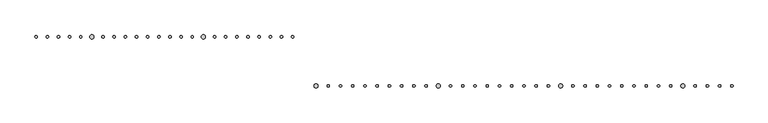
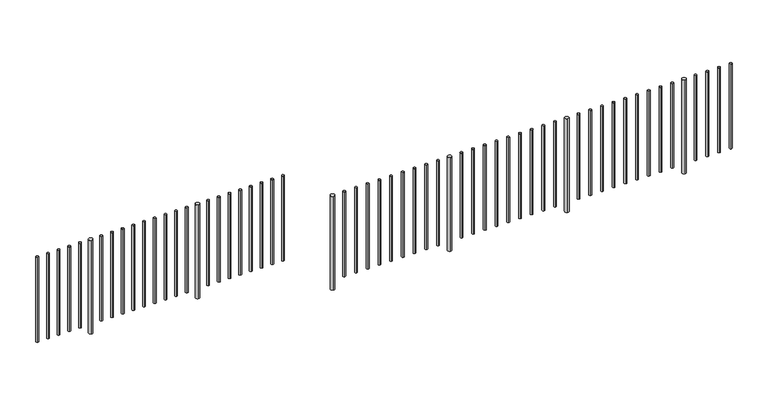
"""IFC4 building model written with IfcOpenShell, lengths in millimetres: railing geometry."""

from ifc_helpers import new_model, si_unit, point, frame, frame_2d, origin, place, context, project, spatial, circle_curve, trimmed, segment, composite_curve, outline, extrude, source, transform, mapped, element, save


def railing_a768a802(model_context):
    return source(origin(), model_context, "Body", "SweptSolid", [
        extrude(outline(composite_curve([segment(trimmed(circle_curve(frame_2d((4462.388051, -8663.7965465)), 12.5), [point((4462.388051, -8676.2965465))], [point((4462.388051, -8651.2965465))], False, "CARTESIAN"), True, "CONTINUOUS"), segment(trimmed(circle_curve(frame_2d((4462.388051, -8663.7965465)), 12.5), [point((4462.388051, -8651.2965465))], [point((4462.388051, -8676.2965465))], False, "CARTESIAN"), True, "CONTINUOUS")], self_intersect=False)), frame((0.0, 0.0, 3500.0), z_axis=(0.0, 0.0, 1.0), x_axis=(1.0, 0.0, 0.0)), (0.0, 0.0, 1.0), 949.2),
        extrude(outline(composite_curve([segment(trimmed(circle_curve(frame_2d((4338.300551, -8663.7965465)), 12.5), [point((4338.300551, -8676.2965465))], [point((4338.300551, -8651.2965465))], False, "CARTESIAN"), True, "CONTINUOUS"), segment(trimmed(circle_curve(frame_2d((4338.300551, -8663.7965465)), 12.5), [point((4338.300551, -8651.2965465))], [point((4338.300551, -8676.2965465))], False, "CARTESIAN"), True, "CONTINUOUS")], self_intersect=False)), frame((0.0, 0.0, 3500.0), z_axis=(0.0, 0.0, 1.0), x_axis=(1.0, 0.0, 0.0)), (0.0, 0.0, 1.0), 949.2),
        extrude(outline(composite_curve([segment(trimmed(circle_curve(frame_2d((4214.213051, -8663.7965465)), 12.5), [point((4214.213051, -8676.2965465))], [point((4214.213051, -8651.2965465))], False, "CARTESIAN"), True, "CONTINUOUS"), segment(trimmed(circle_curve(frame_2d((4214.213051, -8663.7965465)), 12.5), [point((4214.213051, -8651.2965465))], [point((4214.213051, -8676.2965465))], False, "CARTESIAN"), True, "CONTINUOUS")], self_intersect=False)), frame((0.0, 0.0, 3500.0), z_axis=(0.0, 0.0, 1.0), x_axis=(1.0, 0.0, 0.0)), (0.0, 0.0, 1.0), 949.2),
        extrude(outline(composite_curve([segment(trimmed(circle_curve(frame_2d((4090.125551, -8663.7965465)), 12.5), [point((4090.125551, -8676.2965465))], [point((4090.125551, -8651.2965465))], False, "CARTESIAN"), True, "CONTINUOUS"), segment(trimmed(circle_curve(frame_2d((4090.125551, -8663.7965465)), 12.5), [point((4090.125551, -8651.2965465))], [point((4090.125551, -8676.2965465))], False, "CARTESIAN"), True, "CONTINUOUS")], self_intersect=False)), frame((0.0, 0.0, 3500.0), z_axis=(0.0, 0.0, 1.0), x_axis=(1.0, 0.0, 0.0)), (0.0, 0.0, 1.0), 949.2),
        extrude(outline(composite_curve([segment(trimmed(circle_curve(frame_2d((3966.038051, -8663.7965465)), 21.0), [point((3966.038051, -8684.7965465))], [point((3966.038051, -8642.7965465))], False, "CARTESIAN"), True, "CONTINUOUS"), segment(trimmed(circle_curve(frame_2d((3966.038051, -8663.7965465)), 21.0), [point((3966.038051, -8642.7965465))], [point((3966.038051, -8684.7965465))], False, "CARTESIAN"), True, "CONTINUOUS")], self_intersect=False)), frame((0.0, 0.0, 3400.0), z_axis=(0.0, 0.0, 1.0), x_axis=(1.0, 0.0, 0.0)), (0.0, 0.0, 1.0), 1049.2),
        extrude(outline(composite_curve([segment(trimmed(circle_curve(frame_2d((3841.950551, -8663.7965465)), 12.5), [point((3841.950551, -8676.2965465))], [point((3841.950551, -8651.2965465))], False, "CARTESIAN"), True, "CONTINUOUS"), segment(trimmed(circle_curve(frame_2d((3841.950551, -8663.7965465)), 12.5), [point((3841.950551, -8651.2965465))], [point((3841.950551, -8676.2965465))], False, "CARTESIAN"), True, "CONTINUOUS")], self_intersect=False)), frame((0.0, 0.0, 3500.0), z_axis=(0.0, 0.0, 1.0), x_axis=(1.0, 0.0, 0.0)), (0.0, 0.0, 1.0), 949.2),
        extrude(outline(composite_curve([segment(trimmed(circle_curve(frame_2d((3717.863051, -8663.7965465)), 12.5), [point((3717.863051, -8676.2965465))], [point((3717.863051, -8651.2965465))], False, "CARTESIAN"), True, "CONTINUOUS"), segment(trimmed(circle_curve(frame_2d((3717.863051, -8663.7965465)), 12.5), [point((3717.863051, -8651.2965465))], [point((3717.863051, -8676.2965465))], False, "CARTESIAN"), True, "CONTINUOUS")], self_intersect=False)), frame((0.0, 0.0, 3500.0), z_axis=(0.0, 0.0, 1.0), x_axis=(1.0, 0.0, 0.0)), (0.0, 0.0, 1.0), 949.2),
        extrude(outline(composite_curve([segment(trimmed(circle_curve(frame_2d((3593.775551, -8663.7965465)), 12.5), [point((3593.775551, -8676.2965465))], [point((3593.775551, -8651.2965465))], False, "CARTESIAN"), True, "CONTINUOUS"), segment(trimmed(circle_curve(frame_2d((3593.775551, -8663.7965465)), 12.5), [point((3593.775551, -8651.2965465))], [point((3593.775551, -8676.2965465))], False, "CARTESIAN"), True, "CONTINUOUS")], self_intersect=False)), frame((0.0, 0.0, 3500.0), z_axis=(0.0, 0.0, 1.0), x_axis=(1.0, 0.0, 0.0)), (0.0, 0.0, 1.0), 949.2),
        extrude(outline(composite_curve([segment(trimmed(circle_curve(frame_2d((3469.688051, -8663.7965465)), 12.5), [point((3469.688051, -8676.2965465))], [point((3469.688051, -8651.2965465))], False, "CARTESIAN"), True, "CONTINUOUS"), segment(trimmed(circle_curve(frame_2d((3469.688051, -8663.7965465)), 12.5), [point((3469.688051, -8651.2965465))], [point((3469.688051, -8676.2965465))], False, "CARTESIAN"), True, "CONTINUOUS")], self_intersect=False)), frame((0.0, 0.0, 3500.0), z_axis=(0.0, 0.0, 1.0), x_axis=(1.0, 0.0, 0.0)), (0.0, 0.0, 1.0), 949.2),
        extrude(outline(composite_curve([segment(trimmed(circle_curve(frame_2d((3345.600551, -8663.7965465)), 12.5), [point((3345.600551, -8676.2965465))], [point((3345.600551, -8651.2965465))], False, "CARTESIAN"), True, "CONTINUOUS"), segment(trimmed(circle_curve(frame_2d((3345.600551, -8663.7965465)), 12.5), [point((3345.600551, -8651.2965465))], [point((3345.600551, -8676.2965465))], False, "CARTESIAN"), True, "CONTINUOUS")], self_intersect=False)), frame((0.0, 0.0, 3500.0), z_axis=(0.0, 0.0, 1.0), x_axis=(1.0, 0.0, 0.0)), (0.0, 0.0, 1.0), 949.2),
        extrude(outline(composite_curve([segment(trimmed(circle_curve(frame_2d((3221.513051, -8663.7965465)), 12.5), [point((3221.513051, -8676.2965465))], [point((3221.513051, -8651.2965465))], False, "CARTESIAN"), True, "CONTINUOUS"), segment(trimmed(circle_curve(frame_2d((3221.513051, -8663.7965465)), 12.5), [point((3221.513051, -8651.2965465))], [point((3221.513051, -8676.2965465))], False, "CARTESIAN"), True, "CONTINUOUS")], self_intersect=False)), frame((0.0, 0.0, 3500.0), z_axis=(0.0, 0.0, 1.0), x_axis=(1.0, 0.0, 0.0)), (0.0, 0.0, 1.0), 949.2),
        extrude(outline(composite_curve([segment(trimmed(circle_curve(frame_2d((3097.425551, -8663.7965465)), 12.5), [point((3097.425551, -8676.2965465))], [point((3097.425551, -8651.2965465))], False, "CARTESIAN"), True, "CONTINUOUS"), segment(trimmed(circle_curve(frame_2d((3097.425551, -8663.7965465)), 12.5), [point((3097.425551, -8651.2965465))], [point((3097.425551, -8676.2965465))], False, "CARTESIAN"), True, "CONTINUOUS")], self_intersect=False)), frame((0.0, 0.0, 3500.0), z_axis=(0.0, 0.0, 1.0), x_axis=(1.0, 0.0, 0.0)), (0.0, 0.0, 1.0), 949.2),
        extrude(outline(composite_curve([segment(trimmed(circle_curve(frame_2d((2973.338051, -8663.7965465)), 12.5), [point((2973.338051, -8676.2965465))], [point((2973.338051, -8651.2965465))], False, "CARTESIAN"), True, "CONTINUOUS"), segment(trimmed(circle_curve(frame_2d((2973.338051, -8663.7965465)), 12.5), [point((2973.338051, -8651.2965465))], [point((2973.338051, -8676.2965465))], False, "CARTESIAN"), True, "CONTINUOUS")], self_intersect=False)), frame((0.0, 0.0, 3500.0), z_axis=(0.0, 0.0, 1.0), x_axis=(1.0, 0.0, 0.0)), (0.0, 0.0, 1.0), 949.2),
        extrude(outline(composite_curve([segment(trimmed(circle_curve(frame_2d((2849.250551, -8663.7965465)), 12.5), [point((2849.250551, -8676.2965465))], [point((2849.250551, -8651.2965465))], False, "CARTESIAN"), True, "CONTINUOUS"), segment(trimmed(circle_curve(frame_2d((2849.250551, -8663.7965465)), 12.5), [point((2849.250551, -8651.2965465))], [point((2849.250551, -8676.2965465))], False, "CARTESIAN"), True, "CONTINUOUS")], self_intersect=False)), frame((0.0, 0.0, 3500.0), z_axis=(0.0, 0.0, 1.0), x_axis=(1.0, 0.0, 0.0)), (0.0, 0.0, 1.0), 949.2),
        extrude(outline(composite_curve([segment(trimmed(circle_curve(frame_2d((2725.163051, -8663.7965465)), 21.0), [point((2725.163051, -8684.7965465))], [point((2725.163051, -8642.7965465))], False, "CARTESIAN"), True, "CONTINUOUS"), segment(trimmed(circle_curve(frame_2d((2725.163051, -8663.7965465)), 21.0), [point((2725.163051, -8642.7965465))], [point((2725.163051, -8684.7965465))], False, "CARTESIAN"), True, "CONTINUOUS")], self_intersect=False)), frame((0.0, 0.0, 3400.0), z_axis=(0.0, 0.0, 1.0), x_axis=(1.0, 0.0, 0.0)), (0.0, 0.0, 1.0), 1049.2),
        extrude(outline(composite_curve([segment(trimmed(circle_curve(frame_2d((2601.075551, -8663.7965465)), 12.5), [point((2601.075551, -8676.2965465))], [point((2601.075551, -8651.2965465))], False, "CARTESIAN"), True, "CONTINUOUS"), segment(trimmed(circle_curve(frame_2d((2601.075551, -8663.7965465)), 12.5), [point((2601.075551, -8651.2965465))], [point((2601.075551, -8676.2965465))], False, "CARTESIAN"), True, "CONTINUOUS")], self_intersect=False)), frame((0.0, 0.0, 3500.0), z_axis=(0.0, 0.0, 1.0), x_axis=(1.0, 0.0, 0.0)), (0.0, 0.0, 1.0), 949.2),
        extrude(outline(composite_curve([segment(trimmed(circle_curve(frame_2d((2476.988051, -8663.7965465)), 12.5), [point((2476.988051, -8676.2965465))], [point((2476.988051, -8651.2965465))], False, "CARTESIAN"), True, "CONTINUOUS"), segment(trimmed(circle_curve(frame_2d((2476.988051, -8663.7965465)), 12.5), [point((2476.988051, -8651.2965465))], [point((2476.988051, -8676.2965465))], False, "CARTESIAN"), True, "CONTINUOUS")], self_intersect=False)), frame((0.0, 0.0, 3500.0), z_axis=(0.0, 0.0, 1.0), x_axis=(1.0, 0.0, 0.0)), (0.0, 0.0, 1.0), 949.2),
        extrude(outline(composite_curve([segment(trimmed(circle_curve(frame_2d((2352.900551, -8663.7965465)), 12.5), [point((2352.900551, -8676.2965465))], [point((2352.900551, -8651.2965465))], False, "CARTESIAN"), True, "CONTINUOUS"), segment(trimmed(circle_curve(frame_2d((2352.900551, -8663.7965465)), 12.5), [point((2352.900551, -8651.2965465))], [point((2352.900551, -8676.2965465))], False, "CARTESIAN"), True, "CONTINUOUS")], self_intersect=False)), frame((0.0, 0.0, 3500.0), z_axis=(0.0, 0.0, 1.0), x_axis=(1.0, 0.0, 0.0)), (0.0, 0.0, 1.0), 949.2),
        extrude(outline(composite_curve([segment(trimmed(circle_curve(frame_2d((2228.813051, -8663.7965465)), 12.5), [point((2228.813051, -8676.2965465))], [point((2228.813051, -8651.2965465))], False, "CARTESIAN"), True, "CONTINUOUS"), segment(trimmed(circle_curve(frame_2d((2228.813051, -8663.7965465)), 12.5), [point((2228.813051, -8651.2965465))], [point((2228.813051, -8676.2965465))], False, "CARTESIAN"), True, "CONTINUOUS")], self_intersect=False)), frame((0.0, 0.0, 3500.0), z_axis=(0.0, 0.0, 1.0), x_axis=(1.0, 0.0, 0.0)), (0.0, 0.0, 1.0), 949.2),
        extrude(outline(composite_curve([segment(trimmed(circle_curve(frame_2d((2104.725551, -8663.7965465)), 12.5), [point((2104.725551, -8676.2965465))], [point((2104.725551, -8651.2965465))], False, "CARTESIAN"), True, "CONTINUOUS"), segment(trimmed(circle_curve(frame_2d((2104.725551, -8663.7965465)), 12.5), [point((2104.725551, -8651.2965465))], [point((2104.725551, -8676.2965465))], False, "CARTESIAN"), True, "CONTINUOUS")], self_intersect=False)), frame((0.0, 0.0, 3500.0), z_axis=(0.0, 0.0, 1.0), x_axis=(1.0, 0.0, 0.0)), (0.0, 0.0, 1.0), 949.2),
        extrude(outline(composite_curve([segment(trimmed(circle_curve(frame_2d((1980.638051, -8663.7965465)), 12.5), [point((1980.638051, -8676.2965465))], [point((1980.638051, -8651.2965465))], False, "CARTESIAN"), True, "CONTINUOUS"), segment(trimmed(circle_curve(frame_2d((1980.638051, -8663.7965465)), 12.5), [point((1980.638051, -8651.2965465))], [point((1980.638051, -8676.2965465))], False, "CARTESIAN"), True, "CONTINUOUS")], self_intersect=False)), frame((0.0, 0.0, 3500.0), z_axis=(0.0, 0.0, 1.0), x_axis=(1.0, 0.0, 0.0)), (0.0, 0.0, 1.0), 949.2),
        extrude(outline(composite_curve([segment(trimmed(circle_curve(frame_2d((1856.550551, -8663.7965465)), 12.5), [point((1856.550551, -8676.2965465))], [point((1856.550551, -8651.2965465))], False, "CARTESIAN"), True, "CONTINUOUS"), segment(trimmed(circle_curve(frame_2d((1856.550551, -8663.7965465)), 12.5), [point((1856.550551, -8651.2965465))], [point((1856.550551, -8676.2965465))], False, "CARTESIAN"), True, "CONTINUOUS")], self_intersect=False)), frame((0.0, 0.0, 3500.0), z_axis=(0.0, 0.0, 1.0), x_axis=(1.0, 0.0, 0.0)), (0.0, 0.0, 1.0), 949.2),
        extrude(outline(composite_curve([segment(trimmed(circle_curve(frame_2d((1732.463051, -8663.7965465)), 12.5), [point((1732.463051, -8676.2965465))], [point((1732.463051, -8651.2965465))], False, "CARTESIAN"), True, "CONTINUOUS"), segment(trimmed(circle_curve(frame_2d((1732.463051, -8663.7965465)), 12.5), [point((1732.463051, -8651.2965465))], [point((1732.463051, -8676.2965465))], False, "CARTESIAN"), True, "CONTINUOUS")], self_intersect=False)), frame((0.0, 0.0, 3500.0), z_axis=(0.0, 0.0, 1.0), x_axis=(1.0, 0.0, 0.0)), (0.0, 0.0, 1.0), 949.2),
        extrude(outline(composite_curve([segment(trimmed(circle_curve(frame_2d((1608.375551, -8663.7965465)), 12.5), [point((1608.375551, -8676.2965465))], [point((1608.375551, -8651.2965465))], False, "CARTESIAN"), True, "CONTINUOUS"), segment(trimmed(circle_curve(frame_2d((1608.375551, -8663.7965465)), 12.5), [point((1608.375551, -8651.2965465))], [point((1608.375551, -8676.2965465))], False, "CARTESIAN"), True, "CONTINUOUS")], self_intersect=False)), frame((0.0, 0.0, 3500.0), z_axis=(0.0, 0.0, 1.0), x_axis=(1.0, 0.0, 0.0)), (0.0, 0.0, 1.0), 949.2),
        extrude(outline(composite_curve([segment(trimmed(circle_curve(frame_2d((1484.288051, -8663.7965465)), 21.0), [point((1484.288051, -8684.7965465))], [point((1484.288051, -8642.7965465))], False, "CARTESIAN"), True, "CONTINUOUS"), segment(trimmed(circle_curve(frame_2d((1484.288051, -8663.7965465)), 21.0), [point((1484.288051, -8642.7965465))], [point((1484.288051, -8684.7965465))], False, "CARTESIAN"), True, "CONTINUOUS")], self_intersect=False)), frame((0.0, 0.0, 3400.0), z_axis=(0.0, 0.0, 1.0), x_axis=(1.0, 0.0, 0.0)), (0.0, 0.0, 1.0), 1049.2),
        extrude(outline(composite_curve([segment(trimmed(circle_curve(frame_2d((1360.200551, -8663.7965465)), 12.5), [point((1360.200551, -8676.2965465))], [point((1360.200551, -8651.2965465))], False, "CARTESIAN"), True, "CONTINUOUS"), segment(trimmed(circle_curve(frame_2d((1360.200551, -8663.7965465)), 12.5), [point((1360.200551, -8651.2965465))], [point((1360.200551, -8676.2965465))], False, "CARTESIAN"), True, "CONTINUOUS")], self_intersect=False)), frame((0.0, 0.0, 3500.0), z_axis=(0.0, 0.0, 1.0), x_axis=(1.0, 0.0, 0.0)), (0.0, 0.0, 1.0), 949.2),
        extrude(outline(composite_curve([segment(trimmed(circle_curve(frame_2d((1236.113051, -8663.7965465)), 12.5), [point((1236.113051, -8676.2965465))], [point((1236.113051, -8651.2965465))], False, "CARTESIAN"), True, "CONTINUOUS"), segment(trimmed(circle_curve(frame_2d((1236.113051, -8663.7965465)), 12.5), [point((1236.113051, -8651.2965465))], [point((1236.113051, -8676.2965465))], False, "CARTESIAN"), True, "CONTINUOUS")], self_intersect=False)), frame((0.0, 0.0, 3500.0), z_axis=(0.0, 0.0, 1.0), x_axis=(1.0, 0.0, 0.0)), (0.0, 0.0, 1.0), 949.2),
        extrude(outline(composite_curve([segment(trimmed(circle_curve(frame_2d((1112.025551, -8663.7965465)), 12.5), [point((1112.025551, -8676.2965465))], [point((1112.025551, -8651.2965465))], False, "CARTESIAN"), True, "CONTINUOUS"), segment(trimmed(circle_curve(frame_2d((1112.025551, -8663.7965465)), 12.5), [point((1112.025551, -8651.2965465))], [point((1112.025551, -8676.2965465))], False, "CARTESIAN"), True, "CONTINUOUS")], self_intersect=False)), frame((0.0, 0.0, 3500.0), z_axis=(0.0, 0.0, 1.0), x_axis=(1.0, 0.0, 0.0)), (0.0, 0.0, 1.0), 949.2),
        extrude(outline(composite_curve([segment(trimmed(circle_curve(frame_2d((987.938051, -8663.7965465)), 12.5), [point((987.938051, -8676.2965465))], [point((987.938051, -8651.2965465))], False, "CARTESIAN"), True, "CONTINUOUS"), segment(trimmed(circle_curve(frame_2d((987.938051, -8663.7965465)), 12.5), [point((987.938051, -8651.2965465))], [point((987.938051, -8676.2965465))], False, "CARTESIAN"), True, "CONTINUOUS")], self_intersect=False)), frame((0.0, 0.0, 3500.0), z_axis=(0.0, 0.0, 1.0), x_axis=(1.0, 0.0, 0.0)), (0.0, 0.0, 1.0), 949.2),
        extrude(outline(composite_curve([segment(trimmed(circle_curve(frame_2d((863.850551, -8663.7965465)), 12.5), [point((863.850551, -8676.2965465))], [point((863.850551, -8651.2965465))], False, "CARTESIAN"), True, "CONTINUOUS"), segment(trimmed(circle_curve(frame_2d((863.850551, -8663.7965465)), 12.5), [point((863.850551, -8651.2965465))], [point((863.850551, -8676.2965465))], False, "CARTESIAN"), True, "CONTINUOUS")], self_intersect=False)), frame((0.0, 0.0, 3500.0), z_axis=(0.0, 0.0, 1.0), x_axis=(1.0, 0.0, 0.0)), (0.0, 0.0, 1.0), 949.2),
        extrude(outline(composite_curve([segment(trimmed(circle_curve(frame_2d((739.763051, -8663.7965465)), 12.5), [point((739.763051, -8676.2965465))], [point((739.763051, -8651.2965465))], False, "CARTESIAN"), True, "CONTINUOUS"), segment(trimmed(circle_curve(frame_2d((739.763051, -8663.7965465)), 12.5), [point((739.763051, -8651.2965465))], [point((739.763051, -8676.2965465))], False, "CARTESIAN"), True, "CONTINUOUS")], self_intersect=False)), frame((0.0, 0.0, 3500.0), z_axis=(0.0, 0.0, 1.0), x_axis=(1.0, 0.0, 0.0)), (0.0, 0.0, 1.0), 949.2),
        extrude(outline(composite_curve([segment(trimmed(circle_curve(frame_2d((615.675551, -8663.7965465)), 12.5), [point((615.675551, -8676.2965465))], [point((615.675551, -8651.2965465))], False, "CARTESIAN"), True, "CONTINUOUS"), segment(trimmed(circle_curve(frame_2d((615.675551, -8663.7965465)), 12.5), [point((615.675551, -8651.2965465))], [point((615.675551, -8676.2965465))], False, "CARTESIAN"), True, "CONTINUOUS")], self_intersect=False)), frame((0.0, 0.0, 3500.0), z_axis=(0.0, 0.0, 1.0), x_axis=(1.0, 0.0, 0.0)), (0.0, 0.0, 1.0), 949.2),
        extrude(outline(composite_curve([segment(trimmed(circle_curve(frame_2d((491.588051, -8663.7965465)), 12.5), [point((491.588051, -8676.2965465))], [point((491.588051, -8651.2965465))], False, "CARTESIAN"), True, "CONTINUOUS"), segment(trimmed(circle_curve(frame_2d((491.588051, -8663.7965465)), 12.5), [point((491.588051, -8651.2965465))], [point((491.588051, -8676.2965465))], False, "CARTESIAN"), True, "CONTINUOUS")], self_intersect=False)), frame((0.0, 0.0, 3500.0), z_axis=(0.0, 0.0, 1.0), x_axis=(1.0, 0.0, 0.0)), (0.0, 0.0, 1.0), 949.2),
        extrude(outline(composite_curve([segment(trimmed(circle_curve(frame_2d((367.500551, -8663.7965465)), 12.5), [point((367.500551, -8676.2965465))], [point((367.500551, -8651.2965465))], False, "CARTESIAN"), True, "CONTINUOUS"), segment(trimmed(circle_curve(frame_2d((367.500551, -8663.7965465)), 12.5), [point((367.500551, -8651.2965465))], [point((367.500551, -8676.2965465))], False, "CARTESIAN"), True, "CONTINUOUS")], self_intersect=False)), frame((0.0, 0.0, 3500.0), z_axis=(0.0, 0.0, 1.0), x_axis=(1.0, 0.0, 0.0)), (0.0, 0.0, 1.0), 949.2),
        extrude(outline(composite_curve([segment(trimmed(circle_curve(frame_2d((243.413051, -8663.7965465)), 21.0), [point((243.413051, -8684.7965465))], [point((243.413051, -8642.7965465))], False, "CARTESIAN"), True, "CONTINUOUS"), segment(trimmed(circle_curve(frame_2d((243.413051, -8663.7965465)), 21.0), [point((243.413051, -8642.7965465))], [point((243.413051, -8684.7965465))], False, "CARTESIAN"), True, "CONTINUOUS")], self_intersect=False)), frame((0.0, 0.0, 3400.0), z_axis=(0.0, 0.0, 1.0), x_axis=(1.0, 0.0, 0.0)), (0.0, 0.0, 1.0), 1049.2),
        extrude(outline(composite_curve([segment(trimmed(circle_curve(frame_2d((6.185551, -8163.7965465)), 12.5), [point((6.185551, -8176.2965465))], [point((6.185551, -8151.2965465))], False, "CARTESIAN"), True, "CONTINUOUS"), segment(trimmed(circle_curve(frame_2d((6.185551, -8163.7965465)), 12.5), [point((6.185551, -8151.2965465))], [point((6.185551, -8176.2965465))], False, "CARTESIAN"), True, "CONTINUOUS")], self_intersect=False)), frame((0.0, 0.0, 3500.0), z_axis=(0.0, 0.0, 1.0), x_axis=(1.0, 0.0, 0.0)), (0.0, 0.0, 1.0), 949.2),
        extrude(outline(composite_curve([segment(trimmed(circle_curve(frame_2d((-106.954449, -8163.7965465)), 12.5), [point((-106.954449, -8176.2965465))], [point((-106.954449, -8151.2965465))], False, "CARTESIAN"), True, "CONTINUOUS"), segment(trimmed(circle_curve(frame_2d((-106.954449, -8163.7965465)), 12.5), [point((-106.954449, -8151.2965465))], [point((-106.954449, -8176.2965465))], False, "CARTESIAN"), True, "CONTINUOUS")], self_intersect=False)), frame((0.0, 0.0, 3500.0), z_axis=(0.0, 0.0, 1.0), x_axis=(1.0, 0.0, 0.0)), (0.0, 0.0, 1.0), 949.2),
        extrude(outline(composite_curve([segment(trimmed(circle_curve(frame_2d((-220.094449, -8163.7965465)), 12.5), [point((-220.094449, -8176.2965465))], [point((-220.094449, -8151.2965465))], False, "CARTESIAN"), True, "CONTINUOUS"), segment(trimmed(circle_curve(frame_2d((-220.094449, -8163.7965465)), 12.5), [point((-220.094449, -8151.2965465))], [point((-220.094449, -8176.2965465))], False, "CARTESIAN"), True, "CONTINUOUS")], self_intersect=False)), frame((0.0, 0.0, 3500.0), z_axis=(0.0, 0.0, 1.0), x_axis=(1.0, 0.0, 0.0)), (0.0, 0.0, 1.0), 949.2),
        extrude(outline(composite_curve([segment(trimmed(circle_curve(frame_2d((-333.234449, -8163.7965465)), 12.5), [point((-333.234449, -8176.2965465))], [point((-333.234449, -8151.2965465))], False, "CARTESIAN"), True, "CONTINUOUS"), segment(trimmed(circle_curve(frame_2d((-333.234449, -8163.7965465)), 12.5), [point((-333.234449, -8151.2965465))], [point((-333.234449, -8176.2965465))], False, "CARTESIAN"), True, "CONTINUOUS")], self_intersect=False)), frame((0.0, 0.0, 3500.0), z_axis=(0.0, 0.0, 1.0), x_axis=(1.0, 0.0, 0.0)), (0.0, 0.0, 1.0), 949.2),
        extrude(outline(composite_curve([segment(trimmed(circle_curve(frame_2d((-446.374449, -8163.7965465)), 12.5), [point((-446.374449, -8176.2965465))], [point((-446.374449, -8151.2965465))], False, "CARTESIAN"), True, "CONTINUOUS"), segment(trimmed(circle_curve(frame_2d((-446.374449, -8163.7965465)), 12.5), [point((-446.374449, -8151.2965465))], [point((-446.374449, -8176.2965465))], False, "CARTESIAN"), True, "CONTINUOUS")], self_intersect=False)), frame((0.0, 0.0, 3500.0), z_axis=(0.0, 0.0, 1.0), x_axis=(1.0, 0.0, 0.0)), (0.0, 0.0, 1.0), 949.2),
        extrude(outline(composite_curve([segment(trimmed(circle_curve(frame_2d((-559.514449, -8163.7965465)), 12.5), [point((-559.514449, -8176.2965465))], [point((-559.514449, -8151.2965465))], False, "CARTESIAN"), True, "CONTINUOUS"), segment(trimmed(circle_curve(frame_2d((-559.514449, -8163.7965465)), 12.5), [point((-559.514449, -8151.2965465))], [point((-559.514449, -8176.2965465))], False, "CARTESIAN"), True, "CONTINUOUS")], self_intersect=False)), frame((0.0, 0.0, 3500.0), z_axis=(0.0, 0.0, 1.0), x_axis=(1.0, 0.0, 0.0)), (0.0, 0.0, 1.0), 949.2),
        extrude(outline(composite_curve([segment(trimmed(circle_curve(frame_2d((-672.654449, -8163.7965465)), 12.5), [point((-672.654449, -8176.2965465))], [point((-672.654449, -8151.2965465))], False, "CARTESIAN"), True, "CONTINUOUS"), segment(trimmed(circle_curve(frame_2d((-672.654449, -8163.7965465)), 12.5), [point((-672.654449, -8151.2965465))], [point((-672.654449, -8176.2965465))], False, "CARTESIAN"), True, "CONTINUOUS")], self_intersect=False)), frame((0.0, 0.0, 3500.0), z_axis=(0.0, 0.0, 1.0), x_axis=(1.0, 0.0, 0.0)), (0.0, 0.0, 1.0), 949.2),
        extrude(outline(composite_curve([segment(trimmed(circle_curve(frame_2d((-785.794449, -8163.7965465)), 12.5), [point((-785.794449, -8176.2965465))], [point((-785.794449, -8151.2965465))], False, "CARTESIAN"), True, "CONTINUOUS"), segment(trimmed(circle_curve(frame_2d((-785.794449, -8163.7965465)), 12.5), [point((-785.794449, -8151.2965465))], [point((-785.794449, -8176.2965465))], False, "CARTESIAN"), True, "CONTINUOUS")], self_intersect=False)), frame((0.0, 0.0, 3500.0), z_axis=(0.0, 0.0, 1.0), x_axis=(1.0, 0.0, 0.0)), (0.0, 0.0, 1.0), 949.2),
        extrude(outline(composite_curve([segment(trimmed(circle_curve(frame_2d((-898.934449, -8163.7965465)), 21.0), [point((-898.934449, -8184.7965465))], [point((-898.934449, -8142.7965465))], False, "CARTESIAN"), True, "CONTINUOUS"), segment(trimmed(circle_curve(frame_2d((-898.934449, -8163.7965465)), 21.0), [point((-898.934449, -8142.7965465))], [point((-898.934449, -8184.7965465))], False, "CARTESIAN"), True, "CONTINUOUS")], self_intersect=False)), frame((0.0, 0.0, 3400.0), z_axis=(0.0, 0.0, 1.0), x_axis=(1.0, 0.0, 0.0)), (0.0, 0.0, 1.0), 1049.2),
        extrude(outline(composite_curve([segment(trimmed(circle_curve(frame_2d((-1012.074449, -8163.7965465)), 12.5), [point((-1012.074449, -8176.2965465))], [point((-1012.074449, -8151.2965465))], False, "CARTESIAN"), True, "CONTINUOUS"), segment(trimmed(circle_curve(frame_2d((-1012.074449, -8163.7965465)), 12.5), [point((-1012.074449, -8151.2965465))], [point((-1012.074449, -8176.2965465))], False, "CARTESIAN"), True, "CONTINUOUS")], self_intersect=False)), frame((0.0, 0.0, 3500.0), z_axis=(0.0, 0.0, 1.0), x_axis=(1.0, 0.0, 0.0)), (0.0, 0.0, 1.0), 949.2),
        extrude(outline(composite_curve([segment(trimmed(circle_curve(frame_2d((-1125.214449, -8163.7965465)), 12.5), [point((-1125.214449, -8176.2965465))], [point((-1125.214449, -8151.2965465))], False, "CARTESIAN"), True, "CONTINUOUS"), segment(trimmed(circle_curve(frame_2d((-1125.214449, -8163.7965465)), 12.5), [point((-1125.214449, -8151.2965465))], [point((-1125.214449, -8176.2965465))], False, "CARTESIAN"), True, "CONTINUOUS")], self_intersect=False)), frame((0.0, 0.0, 3500.0), z_axis=(0.0, 0.0, 1.0), x_axis=(1.0, 0.0, 0.0)), (0.0, 0.0, 1.0), 949.2),
        extrude(outline(composite_curve([segment(trimmed(circle_curve(frame_2d((-1238.354449, -8163.7965465)), 12.5), [point((-1238.354449, -8176.2965465))], [point((-1238.354449, -8151.2965465))], False, "CARTESIAN"), True, "CONTINUOUS"), segment(trimmed(circle_curve(frame_2d((-1238.354449, -8163.7965465)), 12.5), [point((-1238.354449, -8151.2965465))], [point((-1238.354449, -8176.2965465))], False, "CARTESIAN"), True, "CONTINUOUS")], self_intersect=False)), frame((0.0, 0.0, 3500.0), z_axis=(0.0, 0.0, 1.0), x_axis=(1.0, 0.0, 0.0)), (0.0, 0.0, 1.0), 949.2),
        extrude(outline(composite_curve([segment(trimmed(circle_curve(frame_2d((-1351.494449, -8163.7965465)), 12.5), [point((-1351.494449, -8176.2965465))], [point((-1351.494449, -8151.2965465))], False, "CARTESIAN"), True, "CONTINUOUS"), segment(trimmed(circle_curve(frame_2d((-1351.494449, -8163.7965465)), 12.5), [point((-1351.494449, -8151.2965465))], [point((-1351.494449, -8176.2965465))], False, "CARTESIAN"), True, "CONTINUOUS")], self_intersect=False)), frame((0.0, 0.0, 3500.0), z_axis=(0.0, 0.0, 1.0), x_axis=(1.0, 0.0, 0.0)), (0.0, 0.0, 1.0), 949.2),
        extrude(outline(composite_curve([segment(trimmed(circle_curve(frame_2d((-1464.634449, -8163.7965465)), 12.5), [point((-1464.634449, -8176.2965465))], [point((-1464.634449, -8151.2965465))], False, "CARTESIAN"), True, "CONTINUOUS"), segment(trimmed(circle_curve(frame_2d((-1464.634449, -8163.7965465)), 12.5), [point((-1464.634449, -8151.2965465))], [point((-1464.634449, -8176.2965465))], False, "CARTESIAN"), True, "CONTINUOUS")], self_intersect=False)), frame((0.0, 0.0, 3500.0), z_axis=(0.0, 0.0, 1.0), x_axis=(1.0, 0.0, 0.0)), (0.0, 0.0, 1.0), 949.2),
        extrude(outline(composite_curve([segment(trimmed(circle_curve(frame_2d((-1577.774449, -8163.7965465)), 12.5), [point((-1577.774449, -8176.2965465))], [point((-1577.774449, -8151.2965465))], False, "CARTESIAN"), True, "CONTINUOUS"), segment(trimmed(circle_curve(frame_2d((-1577.774449, -8163.7965465)), 12.5), [point((-1577.774449, -8151.2965465))], [point((-1577.774449, -8176.2965465))], False, "CARTESIAN"), True, "CONTINUOUS")], self_intersect=False)), frame((0.0, 0.0, 3500.0), z_axis=(0.0, 0.0, 1.0), x_axis=(1.0, 0.0, 0.0)), (0.0, 0.0, 1.0), 949.2),
        extrude(outline(composite_curve([segment(trimmed(circle_curve(frame_2d((-1690.914449, -8163.7965465)), 12.5), [point((-1690.914449, -8176.2965465))], [point((-1690.914449, -8151.2965465))], False, "CARTESIAN"), True, "CONTINUOUS"), segment(trimmed(circle_curve(frame_2d((-1690.914449, -8163.7965465)), 12.5), [point((-1690.914449, -8151.2965465))], [point((-1690.914449, -8176.2965465))], False, "CARTESIAN"), True, "CONTINUOUS")], self_intersect=False)), frame((0.0, 0.0, 3500.0), z_axis=(0.0, 0.0, 1.0), x_axis=(1.0, 0.0, 0.0)), (0.0, 0.0, 1.0), 949.2),
        extrude(outline(composite_curve([segment(trimmed(circle_curve(frame_2d((-1804.054449, -8163.7965465)), 12.5), [point((-1804.054449, -8176.2965465))], [point((-1804.054449, -8151.2965465))], False, "CARTESIAN"), True, "CONTINUOUS"), segment(trimmed(circle_curve(frame_2d((-1804.054449, -8163.7965465)), 12.5), [point((-1804.054449, -8151.2965465))], [point((-1804.054449, -8176.2965465))], False, "CARTESIAN"), True, "CONTINUOUS")], self_intersect=False)), frame((0.0, 0.0, 3500.0), z_axis=(0.0, 0.0, 1.0), x_axis=(1.0, 0.0, 0.0)), (0.0, 0.0, 1.0), 949.2),
        extrude(outline(composite_curve([segment(trimmed(circle_curve(frame_2d((-1917.194449, -8163.7965465)), 12.5), [point((-1917.194449, -8176.2965465))], [point((-1917.194449, -8151.2965465))], False, "CARTESIAN"), True, "CONTINUOUS"), segment(trimmed(circle_curve(frame_2d((-1917.194449, -8163.7965465)), 12.5), [point((-1917.194449, -8151.2965465))], [point((-1917.194449, -8176.2965465))], False, "CARTESIAN"), True, "CONTINUOUS")], self_intersect=False)), frame((0.0, 0.0, 3500.0), z_axis=(0.0, 0.0, 1.0), x_axis=(1.0, 0.0, 0.0)), (0.0, 0.0, 1.0), 949.2),
        extrude(outline(composite_curve([segment(trimmed(circle_curve(frame_2d((-2030.334449, -8163.7965465)), 21.0), [point((-2030.334449, -8184.7965465))], [point((-2030.334449, -8142.7965465))], False, "CARTESIAN"), True, "CONTINUOUS"), segment(trimmed(circle_curve(frame_2d((-2030.334449, -8163.7965465)), 21.0), [point((-2030.334449, -8142.7965465))], [point((-2030.334449, -8184.7965465))], False, "CARTESIAN"), True, "CONTINUOUS")], self_intersect=False)), frame((0.0, 0.0, 3400.0), z_axis=(0.0, 0.0, 1.0), x_axis=(1.0, 0.0, 0.0)), (0.0, 0.0, 1.0), 1049.2),
        extrude(outline(composite_curve([segment(trimmed(circle_curve(frame_2d((-2143.474449, -8163.7965465)), 12.5), [point((-2143.474449, -8176.2965465))], [point((-2143.474449, -8151.2965465))], False, "CARTESIAN"), True, "CONTINUOUS"), segment(trimmed(circle_curve(frame_2d((-2143.474449, -8163.7965465)), 12.5), [point((-2143.474449, -8151.2965465))], [point((-2143.474449, -8176.2965465))], False, "CARTESIAN"), True, "CONTINUOUS")], self_intersect=False)), frame((0.0, 0.0, 3500.0), z_axis=(0.0, 0.0, 1.0), x_axis=(1.0, 0.0, 0.0)), (0.0, 0.0, 1.0), 949.2),
        extrude(outline(composite_curve([segment(trimmed(circle_curve(frame_2d((-2256.614449, -8163.7965465)), 12.5), [point((-2256.614449, -8176.2965465))], [point((-2256.614449, -8151.2965465))], False, "CARTESIAN"), True, "CONTINUOUS"), segment(trimmed(circle_curve(frame_2d((-2256.614449, -8163.7965465)), 12.5), [point((-2256.614449, -8151.2965465))], [point((-2256.614449, -8176.2965465))], False, "CARTESIAN"), True, "CONTINUOUS")], self_intersect=False)), frame((0.0, 0.0, 3500.0), z_axis=(0.0, 0.0, 1.0), x_axis=(1.0, 0.0, 0.0)), (0.0, 0.0, 1.0), 949.2),
        extrude(outline(composite_curve([segment(trimmed(circle_curve(frame_2d((-2369.754449, -8163.7965465)), 12.5), [point((-2369.754449, -8176.2965465))], [point((-2369.754449, -8151.2965465))], False, "CARTESIAN"), True, "CONTINUOUS"), segment(trimmed(circle_curve(frame_2d((-2369.754449, -8163.7965465)), 12.5), [point((-2369.754449, -8151.2965465))], [point((-2369.754449, -8176.2965465))], False, "CARTESIAN"), True, "CONTINUOUS")], self_intersect=False)), frame((0.0, 0.0, 3500.0), z_axis=(0.0, 0.0, 1.0), x_axis=(1.0, 0.0, 0.0)), (0.0, 0.0, 1.0), 949.2),
        extrude(outline(composite_curve([segment(trimmed(circle_curve(frame_2d((-2482.894449, -8163.7965465)), 12.5), [point((-2482.894449, -8176.2965465))], [point((-2482.894449, -8151.2965465))], False, "CARTESIAN"), True, "CONTINUOUS"), segment(trimmed(circle_curve(frame_2d((-2482.894449, -8163.7965465)), 12.5), [point((-2482.894449, -8151.2965465))], [point((-2482.894449, -8176.2965465))], False, "CARTESIAN"), True, "CONTINUOUS")], self_intersect=False)), frame((0.0, 0.0, 3500.0), z_axis=(0.0, 0.0, 1.0), x_axis=(1.0, 0.0, 0.0)), (0.0, 0.0, 1.0), 949.2),
        extrude(outline(composite_curve([segment(trimmed(circle_curve(frame_2d((-2596.034449, -8163.7965465)), 12.5), [point((-2596.034449, -8176.2965465))], [point((-2596.034449, -8151.2965465))], False, "CARTESIAN"), True, "CONTINUOUS"), segment(trimmed(circle_curve(frame_2d((-2596.034449, -8163.7965465)), 12.5), [point((-2596.034449, -8151.2965465))], [point((-2596.034449, -8176.2965465))], False, "CARTESIAN"), True, "CONTINUOUS")], self_intersect=False)), frame((0.0, 0.0, 3500.0), z_axis=(0.0, 0.0, 1.0), x_axis=(1.0, 0.0, 0.0)), (0.0, 0.0, 1.0), 949.2),
    ])


if __name__ == "__main__":
    model = new_model("IFC4")
    model_context = context("Model", 3, world=origin())
    ifc_project = project(units=[si_unit("LENGTHUNIT", "METRE", prefix="MILLI")], contexts=[model_context])
    site = spatial("IfcSite", under=ifc_project)
    building = spatial("IfcBuilding", under=site)
    placement = place(None, origin())
    railing_shape = railing_a768a802(model_context)
    element("IfcRailing", 1, at=placement, inside=building, context=model_context, shape_type="MappedRepresentation", body=[
        mapped(railing_shape, transform((0.0, 0.0, 0.0), x_axis=(1.0, 0.0, 0.0), y_axis=(0.0, 1.0, 0.0), z_axis=(0.0, 0.0, 1.0))),
    ])
    save(model, "model.ifc")

# Revit data of these elements
# Element 1 (IfcRailing)
#   Materials on its faces: "Ferro - Pintura Esmalte"
# Materials
#   "Ferro - Pintura Esmalte": class "Pintura", colour RGB 255 255 255, transparency 0, Cost = 0
